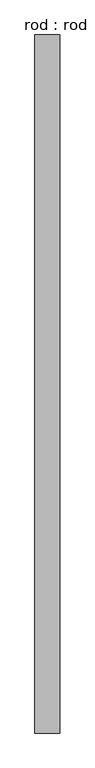
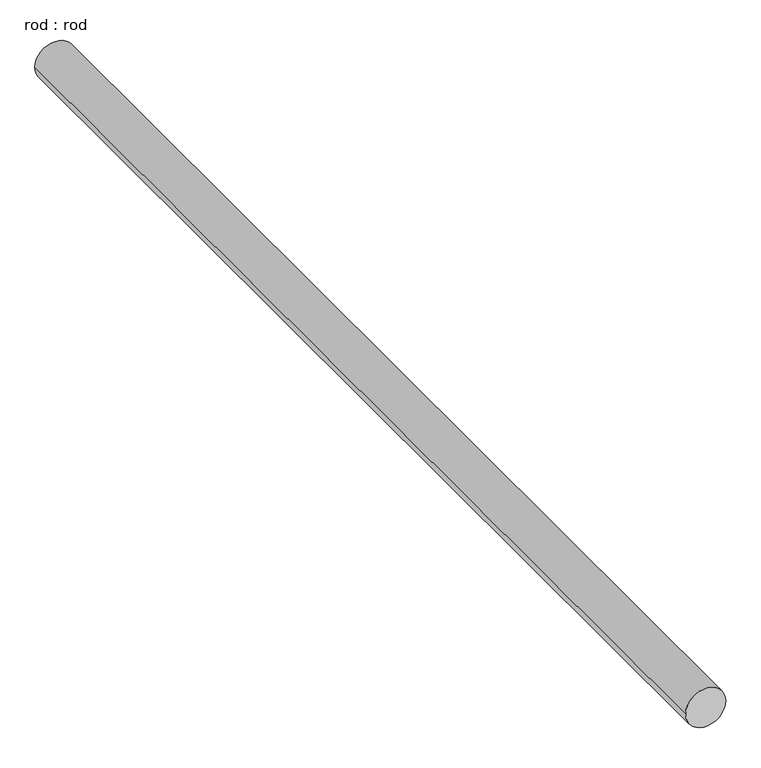
"""IFC4 building model written with IfcOpenShell, lengths in millimetres: proxy geometry, rod : rod."""

import ifcopenshell
import ifcopenshell.guid

model = None  # the IFC model being written
_history = None  # IfcOwnerHistory: only IFC2X3 demands one
_inside = {}  # id of a spatial element -> (the spatial element, [elements in it])
_under = {}  # id of a project, library or spatial element -> (it, [spatial elements below it])
_declared = {}  # id of a project -> (the project, [libraries it declares])
_typed = {}  # id of a type object -> (the type object, [elements of that type])
_made_of = {}  # id of a material, layer set ... -> (it, [elements and type objects made of it])


def new_model(schema):
    """Start an empty IFC model of exactly this schema.

    Asked for "IFC4X3", IfcOpenShell would pick the latest addendum, in which some entities
    have other attributes; the version numbers below select the first issue.
    IFC2X3 requires an IfcOwnerHistory on every rooted entity: one is made here for all.
    """
    global model, _history
    if schema == "IFC4X3":
        model = ifcopenshell.file(schema_version=(4, 3, 0, 0))
    else:
        model = ifcopenshell.file(schema=schema)
    _inside.clear()
    _under.clear()
    _declared.clear()
    _typed.clear()
    _made_of.clear()
    _history = None
    if model.schema == "IFC2X3":
        org = make("IfcOrganization", Name="unknown")
        user = make(
            "IfcPersonAndOrganization",
            ThePerson=make("IfcPerson", FamilyName="unknown"),
            TheOrganization=org,
        )
        app = make(
            "IfcApplication",
            ApplicationDeveloper=org,
            Version="unknown",
            ApplicationFullName="unknown",
            ApplicationIdentifier="unknown",
        )
        _history = make(
            "IfcOwnerHistory",
            OwningUser=user,
            OwningApplication=app,
            ChangeAction="ADDED",
            CreationDate=0,
        )
    return model


def make(cls, **values):
    """One entity of the class cls with the attributes given. An attribute that is None is left unset."""
    return model.create_entity(
        cls, **{name: value for name, value in values.items() if value is not None}
    )


def rooted(cls, **values):
    """An entity with a GlobalId (a new one), such as an element, a storey or a relation."""
    return make(cls, GlobalId=ifcopenshell.guid.new(), OwnerHistory=_history, **values)


def si_unit(unit_type, name, prefix=None):
    """IfcSIUnit, for example si_unit("LENGTHUNIT", "METRE", prefix="MILLI")."""
    return make("IfcSIUnit", UnitType=unit_type, Prefix=prefix, Name=name)


def assignment(units):
    """IfcUnitAssignment: the units of a project."""
    return None if units is None else make("IfcUnitAssignment", Units=units)


def point(xyz):
    """IfcCartesianPoint."""
    return None if xyz is None else make("IfcCartesianPoint", Coordinates=xyz)


def direction(xyz):
    """IfcDirection."""
    return None if xyz is None else make("IfcDirection", DirectionRatios=xyz)


def frame(location, z_axis=None, x_axis=None):
    """IfcAxis2Placement3D, a coordinate frame: its origin and axes. An axis left out is left unset."""
    return make(
        "IfcAxis2Placement3D",
        Location=point(location),
        Axis=direction(z_axis),
        RefDirection=direction(x_axis),
    )


def frame_2d(location, x_axis=None):
    """IfcAxis2Placement2D, a coordinate frame in the plane: its origin and x axis."""
    return make(
        "IfcAxis2Placement2D", Location=point(location), RefDirection=direction(x_axis)
    )


def origin():
    """The frame at (0, 0, 0) with its axes left unset."""
    return frame((0.0, 0.0, 0.0))


def place(relative_to, where):
    """IfcLocalPlacement: puts the frame where relative to a parent placement (None: the world)."""
    return make(
        "IfcLocalPlacement", PlacementRelTo=relative_to, RelativePlacement=where
    )


def context(
    kind, dimensions, precision=None, world=None, true_north=None, identifier=None
):
    """IfcGeometricRepresentationContext, for example the 3D "Model" context."""
    return make(
        "IfcGeometricRepresentationContext",
        ContextIdentifier=identifier,
        ContextType=kind,
        CoordinateSpaceDimension=dimensions,
        Precision=precision,
        WorldCoordinateSystem=world,
        TrueNorth=true_north,
    )


def project(units=None, contexts=None):
    """IfcProject with its units and contexts."""
    return rooted(
        "IfcProject",
        Name="project",
        RepresentationContexts=contexts,
        UnitsInContext=assignment(units),
    )


def spatial(cls, under=None, at=None, **own):
    """A site, building, storey or space (cls), placed at a placement, below another one or the project."""
    s = rooted(cls, ObjectPlacement=at, **own)
    if under is not None:
        _under.setdefault(under.id(), (under, []))[1].append(s)
    return s


def circle_curve(where, radius):
    """IfcCircle in the frame where."""
    return make("IfcCircle", Position=where, Radius=radius)


def trimmed(basis, trim1, trim2, sense, master):
    """IfcTrimmedCurve: the piece of a basis curve between two trims."""
    return make(
        "IfcTrimmedCurve",
        BasisCurve=basis,
        Trim1=trim1,
        Trim2=trim2,
        SenseAgreement=sense,
        MasterRepresentation=master,
    )


def segment(curve, same_sense, transition):
    """IfcCompositeCurveSegment."""
    return make(
        "IfcCompositeCurveSegment",
        Transition=transition,
        SameSense=same_sense,
        ParentCurve=curve,
    )


def composite_curve(segments, self_intersect=None):
    """IfcCompositeCurve: segments joined end to end."""
    return make("IfcCompositeCurve", Segments=segments, SelfIntersect=self_intersect)


def outline(outer, holes=None, kind="AREA"):
    """IfcArbitraryClosedProfileDef: a profile drawn as a closed curve; with holes, ...WithVoids."""
    if holes is None:
        return make("IfcArbitraryClosedProfileDef", ProfileType=kind, OuterCurve=outer)
    return make(
        "IfcArbitraryProfileDefWithVoids",
        ProfileType=kind,
        OuterCurve=outer,
        InnerCurves=holes,
    )


def extrude(swept, where, along, depth):
    """IfcExtrudedAreaSolid: the profile swept, set in the frame where, extruded along a direction by depth."""
    return make(
        "IfcExtrudedAreaSolid",
        SweptArea=swept,
        Position=where,
        ExtrudedDirection=direction(along),
        Depth=depth,
    )


def shape(context_of_items, identifier, shape_type, items):
    """IfcShapeRepresentation: the items that make up one representation, for example the "Body"."""
    return make(
        "IfcShapeRepresentation",
        ContextOfItems=context_of_items,
        RepresentationIdentifier=identifier,
        RepresentationType=shape_type,
        Items=items,
    )


def source(mapping_origin, context_of_items, identifier, shape_type, items):
    """IfcRepresentationMap: a shape defined once, which mapped items show again and again."""
    return make(
        "IfcRepresentationMap",
        MappingOrigin=mapping_origin,
        MappedRepresentation=shape(context_of_items, identifier, shape_type, items),
    )


def transform(
    local_origin,
    x_axis=None,
    y_axis=None,
    z_axis=None,
    scale=None,
    scale2=None,
    scale3=None,
    uniform=True,
):
    """IfcCartesianTransformationOperator3D, or its non-uniform kind. x_axis, y_axis, z_axis: its Axis1, 2, 3."""
    if uniform:
        return make(
            "IfcCartesianTransformationOperator3D",
            Axis1=direction(x_axis),
            Axis2=direction(y_axis),
            LocalOrigin=point(local_origin),
            Scale=scale,
            Axis3=direction(z_axis),
        )
    return make(
        "IfcCartesianTransformationOperator3DnonUniform",
        Axis1=direction(x_axis),
        Axis2=direction(y_axis),
        LocalOrigin=point(local_origin),
        Scale=scale,
        Axis3=direction(z_axis),
        Scale2=scale2,
        Scale3=scale3,
    )


def mapped(mapping_source, mapping_target):
    """IfcMappedItem: shows the shape of a source again, moved by a transform."""
    return make(
        "IfcMappedItem", MappingSource=mapping_source, MappingTarget=mapping_target
    )


def made_of(thing, what):
    """Note that an element or type object is made of a material, layer set ...; save() writes the relation."""
    if what is not None:
        _made_of.setdefault(what.id(), (what, []))[1].append(thing)
    return thing


def element(
    cls,
    number,
    at=None,
    inside=None,
    cuts=None,
    type_object=None,
    material=None,
    context=None,
    identifier="Body",
    shape_type=None,
    held_by="IfcProductDefinitionShape",
    body=None,
    shapes=None,
    **own,
):
    """One element of the class cls, such as IfcWall. Its Tag is "e" and its number.

    at: its placement. inside: the storey or other place that contains it. cuts: it is an
    opening in that element (IfcRelVoidsElement). A single representation is given by context,
    identifier, shape_type and body (its items); several are given by shapes. held_by: the class
    of the entity that holds the representations. save() writes the other relations.
    """
    e = rooted(cls, Tag="e%d" % number, ObjectPlacement=at, **own)
    if body is not None:
        shapes = [shape(context, identifier, shape_type, body)]
    if shapes is not None:
        e.Representation = make(held_by, Representations=shapes)
    if inside is not None:
        _inside.setdefault(inside.id(), (inside, []))[1].append(e)
    if cuts is not None:
        rooted(
            "IfcRelVoidsElement", RelatingBuildingElement=cuts, RelatedOpeningElement=e
        )
    if type_object is not None:
        _typed.setdefault(type_object.id(), (type_object, []))[1].append(e)
    return made_of(e, material)


def aggregate(whole, parts):
    """IfcRelAggregates: a whole, such as a stair, and the parts it consists of."""
    return rooted("IfcRelAggregates", RelatingObject=whole, RelatedObjects=parts)


def save(model, path):
    """Write the relations noted so far, then the file.

    IfcRelAggregates (storeys below a building ...), IfcRelContainedInSpatialStructure (elements
    in a storey), IfcRelDefinesByType, IfcRelAssociatesMaterial and IfcRelDeclares: one each for
    every whole, place, type object, material and project.
    """
    for whole, parts in _under.values():
        aggregate(whole, parts)
    for where, things in _inside.values():
        rooted(
            "IfcRelContainedInSpatialStructure",
            RelatedElements=things,
            RelatingStructure=where,
        )
    for kind, things in _typed.values():
        rooted("IfcRelDefinesByType", RelatedObjects=things, RelatingType=kind)
    for what, things in _made_of.values():
        rooted("IfcRelAssociatesMaterial", RelatedObjects=things, RelatingMaterial=what)
    for by, libraries in _declared.values():
        rooted("IfcRelDeclares", RelatingContext=by, RelatedDefinitions=libraries)
    model.write(path)


def rod_rod_7ca7009a(model_context):
    return source(origin(), model_context, "Body", "SweptSolid", [
        extrude(outline(composite_curve([segment(trimmed(circle_curve(frame_2d((0.0108462, 0.0)), 200.0), [point((0.0108462, 200.0))], [point((0.0108462, -200.0))], False, "CARTESIAN"), True, "CONTINUOUS"), segment(trimmed(circle_curve(frame_2d((0.0108462, 0.0)), 200.0), [point((0.0108462, -200.0))], [point((0.0108462, 200.0))], False, "CARTESIAN"), True, "CONTINUOUS")], self_intersect=False)), frame((0.0, -1518.3824958, 0.0), z_axis=(0.0, 1.0, 0.0), x_axis=(0.0, 0.0, 1.0)), (0.0, 0.0, 1.0), 11222.2222222),
    ])


if __name__ == "__main__":
    model = new_model("IFC4")
    model_context = context("Model", 3, world=origin())
    ifc_project = project(units=[si_unit("LENGTHUNIT", "METRE", prefix="MILLI")], contexts=[model_context])
    site = spatial("IfcSite", under=ifc_project)
    building = spatial("IfcBuilding", under=site)
    placement = place(None, origin())
    rod_rod_shape = rod_rod_7ca7009a(model_context)
    element("IfcBuildingElementProxy", 1, Name="rod : rod", ObjectType="rod : rod", at=placement, inside=building, context=model_context, shape_type="MappedRepresentation", body=[
        mapped(rod_rod_shape, transform((0.0, 0.0, 0.0), x_axis=(1.0, 0.0, 0.0), y_axis=(0.0, 1.0, 0.0), z_axis=(0.0, 0.0, 1.0))),
    ])
    save(model, "model.ifc")

# Revit data of these elements
# Type "rod : rod"
#   Default Elevation = 0
